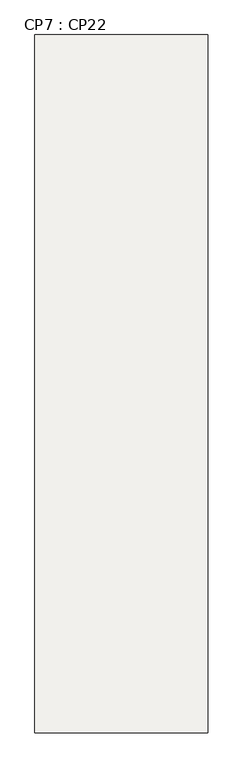
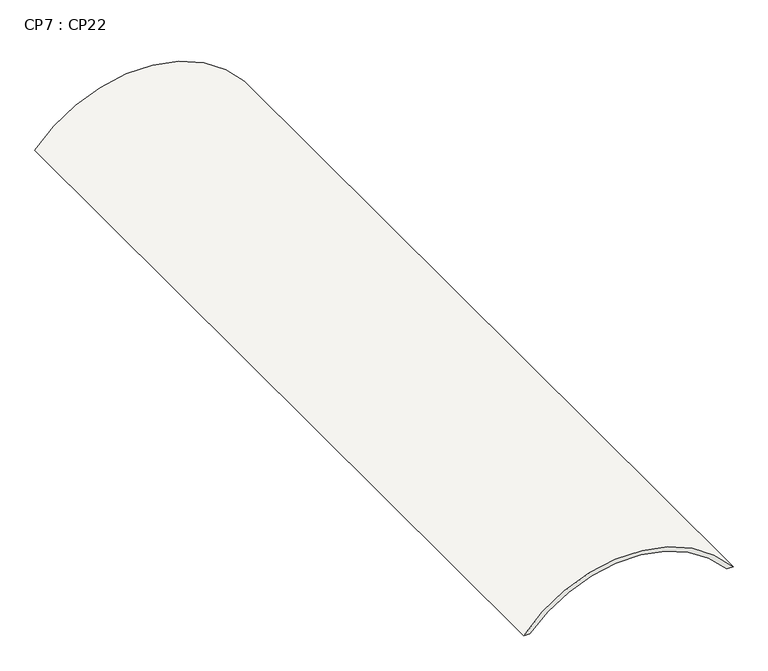
"""IFC4 building model written with IfcOpenShell, lengths in millimetres: slab geometry, CP7 : CP22."""

from ifc_helpers import new_model, si_unit, point, frame, frame_2d, origin, place, context, project, spatial, polyline, circle_curve, trimmed, segment, composite_curve, outline, extrude, source, transform, mapped, element, save


def cp7_cp22_cb3c6a90(model_context):
    return source(origin(), model_context, "Body", "SweptSolid", [
        extrude(outline(composite_curve([segment(trimmed(circle_curve(frame_2d((12562.2036417, 42833.2245513)), 3237.981756), [point((14620.0, 45333.2245512))], [point((14620.0, 40333.2245513))], False, "CARTESIAN"), True, "CONTINUOUS"), segment(polyline([(14620.0, 40333.2245513), (14620.0, 40483.2245513)]), True, "CONTINUOUS"), segment(trimmed(circle_curve(frame_2d((12603.8185575, 42833.2245513)), 3096.3668402), [point((14620.0, 40483.2245513))], [point((14620.0, 45183.2245512))], True, "CARTESIAN"), True, "CONTINUOUS"), segment(polyline([(14620.0, 45183.2245512), (14620.0, 45333.2245512)]), True, "CONTINUOUS")], self_intersect=False)), frame((0.0, -100.2551788, 0.0), z_axis=(0.0, 1.0, 0.0), x_axis=(0.0, 0.0, 1.0)), (0.0, 0.0, 1.0), 20199.9999981),
    ])


if __name__ == "__main__":
    model = new_model("IFC4")
    model_context = context("Model", 3, world=origin())
    ifc_project = project(units=[si_unit("LENGTHUNIT", "METRE", prefix="MILLI")], contexts=[model_context])
    site = spatial("IfcSite", under=ifc_project)
    building = spatial("IfcBuilding", under=site)
    placement = place(None, origin())
    cp7_cp22_shape = cp7_cp22_cb3c6a90(model_context)
    element("IfcSlab", 1, ObjectType="CP7 : CP22", at=placement, inside=building, context=model_context, shape_type="MappedRepresentation", body=[
        mapped(cp7_cp22_shape, transform((0.0, 0.0, 0.0), x_axis=(1.0, 0.0, 0.0), y_axis=(0.0, 1.0, 0.0), z_axis=(0.0, 0.0, 1.0))),
    ])
    save(model, "model.ifc")

# Revit data of these elements
# Element 1 (IfcSlab, "CP7 : CP22")
#   Materials on its faces: "Concrete, RC"
# Materials
#   "Concrete, RC": class "Concrete", colour RGB 128 128 128, transparency 0, Description = "Cast-in-place concrete", Cost = 0
